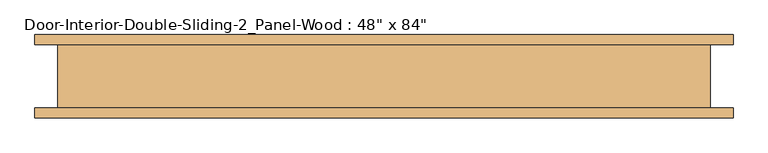
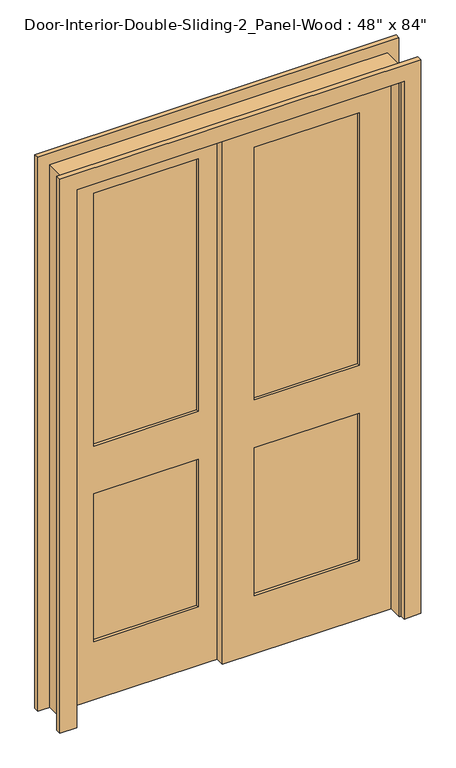
"""IFC4 building model written with IfcOpenShell, lengths in millimetres: door geometry."""

import ifcopenshell
import ifcopenshell.guid

model = None  # the IFC model being written
_history = None  # IfcOwnerHistory: only IFC2X3 demands one
_inside = {}  # id of a spatial element -> (the spatial element, [elements in it])
_under = {}  # id of a project, library or spatial element -> (it, [spatial elements below it])
_declared = {}  # id of a project -> (the project, [libraries it declares])
_typed = {}  # id of a type object -> (the type object, [elements of that type])
_made_of = {}  # id of a material, layer set ... -> (it, [elements and type objects made of it])


def new_model(schema):
    """Start an empty IFC model of exactly this schema.

    Asked for "IFC4X3", IfcOpenShell would pick the latest addendum, in which some entities
    have other attributes; the version numbers below select the first issue.
    IFC2X3 requires an IfcOwnerHistory on every rooted entity: one is made here for all.
    """
    global model, _history
    if schema == "IFC4X3":
        model = ifcopenshell.file(schema_version=(4, 3, 0, 0))
    else:
        model = ifcopenshell.file(schema=schema)
    _inside.clear()
    _under.clear()
    _declared.clear()
    _typed.clear()
    _made_of.clear()
    _history = None
    if model.schema == "IFC2X3":
        org = make("IfcOrganization", Name="unknown")
        user = make(
            "IfcPersonAndOrganization",
            ThePerson=make("IfcPerson", FamilyName="unknown"),
            TheOrganization=org,
        )
        app = make(
            "IfcApplication",
            ApplicationDeveloper=org,
            Version="unknown",
            ApplicationFullName="unknown",
            ApplicationIdentifier="unknown",
        )
        _history = make(
            "IfcOwnerHistory",
            OwningUser=user,
            OwningApplication=app,
            ChangeAction="ADDED",
            CreationDate=0,
        )
    return model


def make(cls, **values):
    """One entity of the class cls with the attributes given. An attribute that is None is left unset."""
    return model.create_entity(
        cls, **{name: value for name, value in values.items() if value is not None}
    )


def rooted(cls, **values):
    """An entity with a GlobalId (a new one), such as an element, a storey or a relation."""
    return make(cls, GlobalId=ifcopenshell.guid.new(), OwnerHistory=_history, **values)


def si_unit(unit_type, name, prefix=None):
    """IfcSIUnit, for example si_unit("LENGTHUNIT", "METRE", prefix="MILLI")."""
    return make("IfcSIUnit", UnitType=unit_type, Prefix=prefix, Name=name)


def assignment(units):
    """IfcUnitAssignment: the units of a project."""
    return None if units is None else make("IfcUnitAssignment", Units=units)


def point(xyz):
    """IfcCartesianPoint."""
    return None if xyz is None else make("IfcCartesianPoint", Coordinates=xyz)


def direction(xyz):
    """IfcDirection."""
    return None if xyz is None else make("IfcDirection", DirectionRatios=xyz)


def frame(location, z_axis=None, x_axis=None):
    """IfcAxis2Placement3D, a coordinate frame: its origin and axes. An axis left out is left unset."""
    return make(
        "IfcAxis2Placement3D",
        Location=point(location),
        Axis=direction(z_axis),
        RefDirection=direction(x_axis),
    )


def origin():
    """The frame at (0, 0, 0) with its axes left unset."""
    return frame((0.0, 0.0, 0.0))


def place(relative_to, where):
    """IfcLocalPlacement: puts the frame where relative to a parent placement (None: the world)."""
    return make(
        "IfcLocalPlacement", PlacementRelTo=relative_to, RelativePlacement=where
    )


def context(
    kind, dimensions, precision=None, world=None, true_north=None, identifier=None
):
    """IfcGeometricRepresentationContext, for example the 3D "Model" context."""
    return make(
        "IfcGeometricRepresentationContext",
        ContextIdentifier=identifier,
        ContextType=kind,
        CoordinateSpaceDimension=dimensions,
        Precision=precision,
        WorldCoordinateSystem=world,
        TrueNorth=true_north,
    )


def project(units=None, contexts=None):
    """IfcProject with its units and contexts."""
    return rooted(
        "IfcProject",
        Name="project",
        RepresentationContexts=contexts,
        UnitsInContext=assignment(units),
    )


def spatial(cls, under=None, at=None, **own):
    """A site, building, storey or space (cls), placed at a placement, below another one or the project."""
    s = rooted(cls, ObjectPlacement=at, **own)
    if under is not None:
        _under.setdefault(under.id(), (under, []))[1].append(s)
    return s


def polyline(points):
    """IfcPolyline through the points."""
    return make("IfcPolyline", Points=[point(p) for p in points])


def outline(outer, holes=None, kind="AREA"):
    """IfcArbitraryClosedProfileDef: a profile drawn as a closed curve; with holes, ...WithVoids."""
    if holes is None:
        return make("IfcArbitraryClosedProfileDef", ProfileType=kind, OuterCurve=outer)
    return make(
        "IfcArbitraryProfileDefWithVoids",
        ProfileType=kind,
        OuterCurve=outer,
        InnerCurves=holes,
    )


def extrude(swept, where, along, depth):
    """IfcExtrudedAreaSolid: the profile swept, set in the frame where, extruded along a direction by depth."""
    return make(
        "IfcExtrudedAreaSolid",
        SweptArea=swept,
        Position=where,
        ExtrudedDirection=direction(along),
        Depth=depth,
    )


def shape(context_of_items, identifier, shape_type, items):
    """IfcShapeRepresentation: the items that make up one representation, for example the "Body"."""
    return make(
        "IfcShapeRepresentation",
        ContextOfItems=context_of_items,
        RepresentationIdentifier=identifier,
        RepresentationType=shape_type,
        Items=items,
    )


def source(mapping_origin, context_of_items, identifier, shape_type, items):
    """IfcRepresentationMap: a shape defined once, which mapped items show again and again."""
    return make(
        "IfcRepresentationMap",
        MappingOrigin=mapping_origin,
        MappedRepresentation=shape(context_of_items, identifier, shape_type, items),
    )


def transform(
    local_origin,
    x_axis=None,
    y_axis=None,
    z_axis=None,
    scale=None,
    scale2=None,
    scale3=None,
    uniform=True,
):
    """IfcCartesianTransformationOperator3D, or its non-uniform kind. x_axis, y_axis, z_axis: its Axis1, 2, 3."""
    if uniform:
        return make(
            "IfcCartesianTransformationOperator3D",
            Axis1=direction(x_axis),
            Axis2=direction(y_axis),
            LocalOrigin=point(local_origin),
            Scale=scale,
            Axis3=direction(z_axis),
        )
    return make(
        "IfcCartesianTransformationOperator3DnonUniform",
        Axis1=direction(x_axis),
        Axis2=direction(y_axis),
        LocalOrigin=point(local_origin),
        Scale=scale,
        Axis3=direction(z_axis),
        Scale2=scale2,
        Scale3=scale3,
    )


def mapped(mapping_source, mapping_target):
    """IfcMappedItem: shows the shape of a source again, moved by a transform."""
    return make(
        "IfcMappedItem", MappingSource=mapping_source, MappingTarget=mapping_target
    )


def made_of(thing, what):
    """Note that an element or type object is made of a material, layer set ...; save() writes the relation."""
    if what is not None:
        _made_of.setdefault(what.id(), (what, []))[1].append(thing)
    return thing


def element(
    cls,
    number,
    at=None,
    inside=None,
    cuts=None,
    type_object=None,
    material=None,
    context=None,
    identifier="Body",
    shape_type=None,
    held_by="IfcProductDefinitionShape",
    body=None,
    shapes=None,
    **own,
):
    """One element of the class cls, such as IfcWall. Its Tag is "e" and its number.

    at: its placement. inside: the storey or other place that contains it. cuts: it is an
    opening in that element (IfcRelVoidsElement). A single representation is given by context,
    identifier, shape_type and body (its items); several are given by shapes. held_by: the class
    of the entity that holds the representations. save() writes the other relations.
    """
    e = rooted(cls, Tag="e%d" % number, ObjectPlacement=at, **own)
    if body is not None:
        shapes = [shape(context, identifier, shape_type, body)]
    if shapes is not None:
        e.Representation = make(held_by, Representations=shapes)
    if inside is not None:
        _inside.setdefault(inside.id(), (inside, []))[1].append(e)
    if cuts is not None:
        rooted(
            "IfcRelVoidsElement", RelatingBuildingElement=cuts, RelatedOpeningElement=e
        )
    if type_object is not None:
        _typed.setdefault(type_object.id(), (type_object, []))[1].append(e)
    return made_of(e, material)


def aggregate(whole, parts):
    """IfcRelAggregates: a whole, such as a stair, and the parts it consists of."""
    return rooted("IfcRelAggregates", RelatingObject=whole, RelatedObjects=parts)


def save(model, path):
    """Write the relations noted so far, then the file.

    IfcRelAggregates (storeys below a building ...), IfcRelContainedInSpatialStructure (elements
    in a storey), IfcRelDefinesByType, IfcRelAssociatesMaterial and IfcRelDeclares: one each for
    every whole, place, type object, material and project.
    """
    for whole, parts in _under.values():
        aggregate(whole, parts)
    for where, things in _inside.values():
        rooted(
            "IfcRelContainedInSpatialStructure",
            RelatedElements=things,
            RelatingStructure=where,
        )
    for kind, things in _typed.values():
        rooted("IfcRelDefinesByType", RelatedObjects=things, RelatingType=kind)
    for what, things in _made_of.values():
        rooted("IfcRelAssociatesMaterial", RelatedObjects=things, RelatingMaterial=what)
    for by, libraries in _declared.values():
        rooted("IfcRelDeclares", RelatingContext=by, RelatedDefinitions=libraries)
    model.write(path)


def door_f0c8ed54(model_context):
    return source(origin(), model_context, "Body", "SweptSolid", [
        extrude(outline(polyline([(488.95, 0.5291667), (95.25, 0.5291667), (95.25, 12.1708333), (488.95, 12.1708333), (488.95, 0.5291667)])), frame((0.0, 0.0, 1009.65), z_axis=(0.0, 0.0, 1.0), x_axis=(1.0, 0.0, 0.0)), (0.0, 0.0, 1.0), 1004.8875),
        extrude(outline(polyline([(488.95, 0.5291667), (95.25, 0.5291667), (95.25, 12.1708333), (488.95, 12.1708333), (488.95, 0.5291667)])), frame((0.0, 0.0, 231.775), z_axis=(0.0, 0.0, 1.0), x_axis=(1.0, 0.0, 0.0)), (0.0, 0.0, 1.0), 587.375),
        extrude(outline(polyline([(2133.6, -25.4), (0.0, -25.4), (0.0, 609.6), (2133.6, 609.6), (2133.6, -25.4)]), holes=[polyline([(2014.5375, 95.25), (2014.5375, 488.95), (1009.65, 488.95), (1009.65, 95.25), (2014.5375, 95.25)]), polyline([(819.15, 95.25), (819.15, 488.95), (231.775, 488.95), (231.775, 95.25), (819.15, 95.25)])]), frame((0.0, -11.1125, 0.0), z_axis=(0.0, 1.0, 0.0), x_axis=(0.0, 0.0, 1.0)), (0.0, 0.0, 1.0), 34.925),
        extrude(outline(polyline([(-95.25, 35.4541667), (-488.95, 35.4541667), (-488.95, 47.0958333), (-95.25, 47.0958333), (-95.25, 35.4541667)])), frame((0.0, 0.0, 1009.65), z_axis=(0.0, 0.0, 1.0), x_axis=(1.0, 0.0, 0.0)), (0.0, 0.0, 1.0), 1004.8875),
        extrude(outline(polyline([(-95.25, 35.4541667), (-488.95, 35.4541667), (-488.95, 47.0958333), (-95.25, 47.0958333), (-95.25, 35.4541667)])), frame((0.0, 0.0, 231.775), z_axis=(0.0, 0.0, 1.0), x_axis=(1.0, 0.0, 0.0)), (0.0, 0.0, 1.0), 587.375),
        extrude(outline(polyline([(2133.6, -609.6), (0.0, -609.6), (0.0, 25.4), (2133.6, 25.4), (2133.6, -609.6)]), holes=[polyline([(2014.5375, -488.95), (2014.5375, -95.25), (1009.65, -95.25), (1009.65, -488.95), (2014.5375, -488.95)]), polyline([(819.15, -488.95), (819.15, -95.25), (231.775, -95.25), (231.775, -488.95), (819.15, -488.95)])]), frame((0.0, 23.8125, 0.0), z_axis=(0.0, 1.0, 0.0), x_axis=(0.0, 0.0, 1.0)), (0.0, 0.0, 1.0), 34.925),
        extrude(outline(polyline([(0.0, 609.6), (0.0, 635.0), (2159.0, 635.0), (2159.0, -635.0), (0.0, -635.0), (0.0, -609.6), (2133.6, -609.6), (2133.6, 609.6), (0.0, 609.6)])), frame((0.0, -65.0875, 0.0), z_axis=(0.0, 1.0, 0.0), x_axis=(0.0, 0.0, 1.0)), (0.0, 0.0, 1.0), 123.825),
        extrude(outline(polyline([(0.0, 615.95), (0.0, 679.45), (2203.45, 679.45), (2203.45, -679.45), (0.0, -679.45), (0.0, -615.95), (2139.95, -615.95), (2139.95, 615.95), (0.0, 615.95)])), frame((0.0, -84.1375, 0.0), z_axis=(0.0, 1.0, 0.0), x_axis=(0.0, 0.0, 1.0)), (0.0, 0.0, 1.0), 19.05),
        extrude(outline(polyline([(0.0, 615.95), (0.0, 679.45), (2203.45, 679.45), (2203.45, -679.45), (0.0, -679.45), (0.0, -615.95), (2139.95, -615.95), (2139.95, 615.95), (0.0, 615.95)])), frame((0.0, 58.7375, 0.0), z_axis=(0.0, 1.0, 0.0), x_axis=(0.0, 0.0, 1.0)), (0.0, 0.0, 1.0), 19.05),
    ])


if __name__ == "__main__":
    model = new_model("IFC4")
    model_context = context("Model", 3, world=origin())
    ifc_project = project(units=[si_unit("LENGTHUNIT", "METRE", prefix="MILLI")], contexts=[model_context])
    site = spatial("IfcSite", under=ifc_project)
    building = spatial("IfcBuilding", under=site)
    placement = place(None, origin())
    door_shape = door_f0c8ed54(model_context)
    element("IfcDoor", 1, ObjectType="Door-Interior-Double-Sliding-2_Panel-Wood : 48\" x 84\"", at=placement, inside=building, context=model_context, shape_type="MappedRepresentation", body=[
        mapped(door_shape, transform((0.0, 0.0, 0.0), x_axis=(1.0, 0.0, 0.0), y_axis=(0.0, 1.0, 0.0), z_axis=(0.0, 0.0, 1.0))),
    ])
    save(model, "model.ifc")

# Revit data of these elements
# Type "Door-Interior-Double-Sliding-2_Panel-Wood : 48\" x 84\""
#   Type Mark = "21"
#   Assembly Code = "C1020300"
#   Analytic Construction = "Wooden"
#   Top Rail = 0' - 4 11/16"
#   Thickness = 0' - 1 3/8"
#   Thermal Resistance (R) = 2.5876 (h·ft²·°F)/BTU
#   Stiles = 0' - 4 3/4"
#   Rough Width = 4' - 2"
#   Rough Height = 7' - 1"
#   Lock Rail = 0' - 7 1/2"
#   Height = 7' - 0"
#   Width = 4' - 0"
#   Heat Transfer Coefficient (U) = 0.3865 BTU/(h·ft²·°F)
#   Bottom Rail = 0' - 9 1/8"
#   Trim Material = Cherry
#   Panel Material = Cherry
#   Frame Material = Cherry
#   Visual Light Transmittance = 0
#   Solar Heat Gain Coefficient = 0
#   Wall Closure = (empty or 0)
#   Function = (empty or 0)
# Element 1 (IfcDoor, "Door-Interior-Double-Sliding-2_Panel-Wood : 48\" x 84\"")
#   Materials on its faces: "Cherry"
# Materials
#   "Cherry": class "Wood", colour RGB 226 177 128, transparency 0, Description = "Prunus Serotina", Cost = 0
